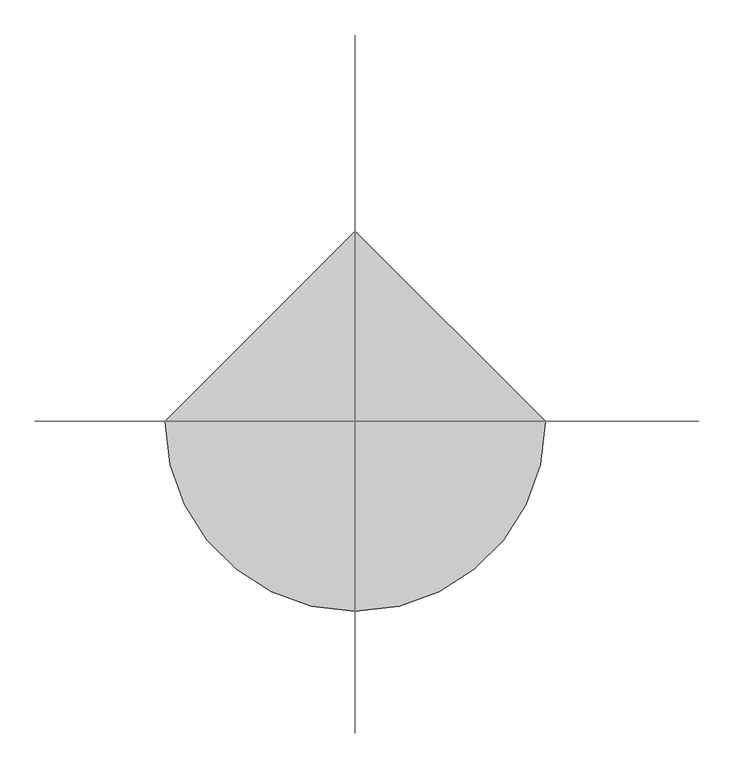
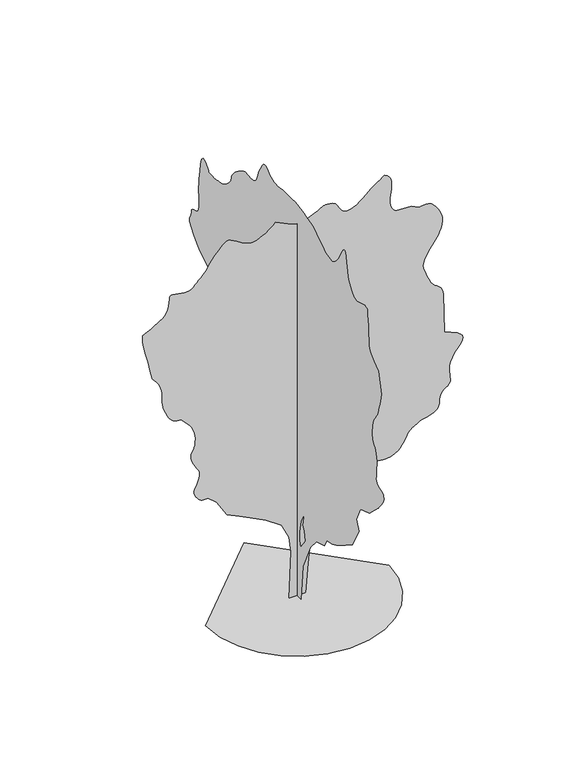
"""IFC4 building model written with IfcOpenShell, lengths in millimetres: geographic element geometry, RPC 木 - 落葉樹 : アメリカサイカチ - 7.6 メートル."""

from ifc_helpers import new_model, si_unit, origin, place, context, project, spatial, triangles, source, transform, mapped, element, save


def geographic_element_4d039a6d(model_context):
    return source(origin(), model_context, "Body", "Tessellation", [
        triangles([(0.0017518, 137.8833715, 0.0), (0.0017518, -126.6771787, 0.0), (0.0017518, -184.1906286, 667.1526644), (0.0017518, -425.7465056, 1173.2690826), (0.0017518, -609.7879246, 1391.8195507), (0.0017518, -862.844862, 1472.3389091), (0.0017518, -931.8629602, 1610.3700188), (0.0017518, -1115.9043428, 1656.3802917), (0.0017518, -1165.0661676, 1674.6229282), (0.0017518, -1231.7358627, 1707.9563587), (0.0017518, -1312.9923855, 1753.8679459), (0.0017518, -1405.9175274, 1809.8393841), (0.0017518, -1507.5978035, 1873.3551292), (0.0017518, -1615.1123165, 1941.9019627), (0.0017518, -1725.5454014, 2012.9618694), (0.0017518, -1932.5919205, 2392.5485836), (0.0017518, -1852.072562, 2576.5999947), (0.0017518, -1978.6023388, 2841.1559395), (0.0017518, -2266.1682163, 2944.6676445), (0.0017518, -2530.7289574, 3197.7222565), (0.0017518, -2537.2320488, 3205.5755562), (0.0017518, -2554.6106392, 3226.7033363), (0.0017518, -2579.6146362, 3257.4834343), (0.0017518, -2609.0773727, 3294.3181046), (0.0017518, -2639.7307343, 3333.559314), (0.0017518, -2668.3574753, 3371.5846092), (0.0017518, -2691.7653488, 3404.7712463), (0.0017518, -2707.3199226, 3435.5004753), (0.0017518, -2714.843882, 3467.42062), (0.0017518, -2714.6918564, 3498.9605553), (0.0017518, -2707.3199226, 3528.4485809), (0.0017518, -2693.1079994, 3554.3391518), (0.0017518, -2672.4612946, 3575.0111458), (0.0017518, -2645.7600174, 3588.8178612), (0.0017518, -2614.4732643, 3598.8750961), (0.0017518, -2581.3627853, 3610.1482452), (0.0017518, -2548.8601181, 3623.8285149), (0.0017518, -2519.3950562, 3641.1309471), (0.0017518, -2495.3485588, 3663.2723282), (0.0017518, -2479.1504196, 3691.4429924), (0.0017518, -2473.2147354, 3726.8588539), (0.0017518, -2475.0617157, 3770.3056206), (0.0017518, -2479.5204552, 3821.0228737), (0.0017518, -2484.9872726, 3877.7694099), (0.0017518, -2489.8486038, 3939.3293152), (0.0017518, -2492.4984421, 4004.5372536), (0.0017518, -2491.3255486, 4072.1267326), (0.0017518, -2484.7186844, 4140.9571243), (0.0017518, -2471.0692268, 4202.6943443), (0.0017518, -2451.5852417, 4251.7396065), (0.0017518, -2428.8815403, 4290.9558174), (0.0017518, -2405.5749687, 4323.1035645), (0.0017518, -2384.2797569, 4351.0463356), (0.0017518, -2367.6128963, 4377.570298), (0.0017518, -2358.1889076, 4405.5130692), (0.0017518, -2353.3934155, 4438.4462334), (0.0017518, -2349.4033974, 4477.4089714), (0.0017518, -2347.022002, 4521.4126808), (0.0017518, -2347.0549942, 4569.4446327), (0.0017518, -2350.307848, 4620.465937), (0.0017518, -2357.5860374, 4673.5138618), (0.0017518, -2369.6928566, 4727.5753876), (0.0017518, -2385.7895485, 4775.3791557), (0.0017518, -2404.1004948, 4812.695192), (0.0017518, -2424.0200638, 4843.1712387), (0.0017518, -2444.9455307, 4870.4550385), (0.0017518, -2466.2735893, 4898.1190475), (0.0017518, -2487.4013695, 4929.8112991), (0.0017518, -2507.7239662, 4969.1280853), (0.0017518, -2527.4434021, 5018.1989273), (0.0017518, -2547.162838, 5075.7053009), (0.0017518, -2566.8721001, 5140.2804291), (0.0017518, -2586.6066513, 5210.4534714), (0.0017518, -2606.3162041, 5284.8826492), (0.0017518, -2626.0254662, 5362.0988663), (0.0017518, -2645.7600174, 5440.7585999), (0.0017518, -2542.2227325, 5820.3272919), (0.0017518, -2404.1993259, 5923.8645767), (0.0017518, -2369.9284527, 5951.1995361), (0.0017518, -2337.0635983, 5979.8262772), (0.0017518, -2307.015723, 6011.0871597), (0.0017518, -2281.193462, 6046.2751282), (0.0017518, -2261.0053047, 6086.6819641), (0.0017518, -2247.8574154, 6133.6244476), (0.0017518, -2243.1630798, 6188.4205215), (0.0017518, -2241.8229, 6252.9444901), (0.0017518, -2238.0660072, 6327.120195), (0.0017518, -2232.2976093, 6409.3523849), (0.0017518, -2224.9205887, 6498.0190659), (0.0017518, -2216.3350662, 6591.5238235), (0.0017518, -2206.9440697, 6688.2214096), (0.0017518, -2197.1528069, 6786.5654068), (0.0017518, -2179.7816288, 6796.2427231), (0.0017518, -2161.706424, 6804.9317276), (0.0017518, -2142.2225842, 6811.6196915), (0.0017518, -2120.6259373, 6815.2677246), (0.0017518, -2096.2121658, 6814.8880966), (0.0017518, -2068.2770977, 6809.4919144), (0.0017518, -2036.1165607, 6798.066449), (0.0017518, -2001.6074753, 6783.4743164), (0.0017518, -1967.1010059, 6770.0983887), (0.0017518, -1932.5919205, 6759.1292908), (0.0017518, -1898.082835, 6751.7826462), (0.0017518, -1863.5763657, 6749.2746597), (0.0017518, -1829.0674255, 6752.7959564), (0.0017518, -1794.5608109, 6763.5627411), (0.0017518, -1761.0576233, 6783.7027908), (0.0017518, -1729.3681332, 6813.5195755), (0.0017518, -1699.1859638, 6851.3934265), (0.0017518, -1670.2098255, 6895.6756073), (0.0017518, -1642.1404633, 6944.8226074), (0.0017518, -1614.6765873, 6997.1612732), (0.0017518, -1587.5116756, 7051.1207703), (0.0017518, -1518.4962662, 7465.2193314), (0.0017518, -1506.0550198, 7474.5925964), (0.0017518, -1492.9096012, 7481.1794037), (0.0017518, -1478.3555477, 7482.1165558), (0.0017518, -1461.6888325, 7474.5925964), (0.0017518, -1442.2049927, 7455.8204865), (0.0017518, -1419.1997108, 7422.9631897), (0.0017518, -1391.9689602, 7373.1830887), (0.0017518, -1362.8939907, 7316.7406036), (0.0017518, -1334.019009, 7265.3396713), (0.0017518, -1304.1384201, 7218.371608), (0.0017518, -1272.0461929, 7175.2033127), (0.0017518, -1236.5315002, 7135.2528442), (0.0017518, -1196.3882383, 7097.9370987), (0.0017518, -1150.4133556, 7062.6223938), (0.0017518, -1098.0975809, 7039.1889404), (0.0017518, -1040.3503063, 7035.6676437), (0.0017518, -978.073439, 7048.7395203), (0.0017518, -912.1764439, 7075.0861679), (0.0017518, -843.5636988, 7111.414183), (0.0017518, -773.1396544, 7154.3795837), (0.0017518, -701.8086159, 7200.6633865), (0.0017518, -657.5437305, 7232.507373), (0.0017518, -613.8792446, 7263.2618912), (0.0017518, -571.4231515, 7291.8124741), (0.0017518, -530.778394, 7317.019075), (0.0017518, -492.5479151, 7337.8178055), (0.0017518, -457.3371283, 7353.0686188), (0.0017518, -425.7465056, 7361.6820465), (0.0017518, -378.7962828, 7372.2459366), (0.0017518, -303.6779573, 7391.2715195), (0.0017518, -210.2471958, 7414.5020782), (0.0017518, -108.3667684, 7437.7576355), (0.0017518, -7.8945933, 7456.7576385), (0.0017518, 81.3095355, 7467.32211), (0.0017518, 149.3864666, 7465.2193314), (0.0017518, 203.5460423, 7458.5057877), (0.0017518, 257.3028083, 7456.6314835), (0.0017518, 310.2544999, 7457.365741), (0.0017518, 362.0002876, 7458.5057877), (0.0017518, 412.1349092, 7457.8471069), (0.0017518, 460.2580619, 7453.1351852), (0.0017518, 505.9669724, 7442.2166656), (0.0017518, 554.0242498, 7432.1085617), (0.0017518, 607.3128576, 7430.4621506), (0.0017518, 662.6104271, 7435.8833313), (0.0017518, 716.7045816, 7446.9030075), (0.0017518, 766.3705908, 7462.1538208), (0.0017518, 808.3909184, 7480.2416702), (0.0017518, 839.5433046, 7499.7230392), (0.0017518, 867.4124611, 7523.4099655), (0.0017518, 900.5129843, 7551.0989731), (0.0017518, 937.0309587, 7576.9898346), (0.0017518, 975.1626429, 7595.2300003), (0.0017518, 1013.0891069, 7599.9925003), (0.0017518, 1049.006682, 7585.4259476), (0.0017518, 1081.0989092, 7545.7283707), (0.0017518, 1108.6666306, 7497.2656311), (0.0017518, 1132.6091372, 7458.075), (0.0017518, 1153.5370022, 7424.7113388), (0.0017518, 1172.0480089, 7393.7539261), (0.0017518, 1188.7477163, 7361.7832031), (0.0017518, 1204.2416107, 7325.4046097), (0.0017518, 1219.1324896, 7281.1730072), (0.0017518, 1233.4508743, 7235.9275131), (0.0017518, 1247.7718025, 7198.1304016), (0.0017518, 1263.4987495, 7166.7927795), (0.0017518, 1282.0426758, 7140.8513397), (0.0017518, 1304.8148323, 7119.3689301), (0.0017518, 1333.2184765, 7101.2810806), (0.0017518, 1368.6648594, 7085.6250595), (0.0017518, 1409.9809422, 7076.5302658), (0.0017518, 1454.1141495, 7076.3023727), (0.0017518, 1499.6558464, 7081.0904526), (0.0017518, 1545.1949272, 7087.0941559), (0.0017518, 1589.3281345, 7090.4887161), (0.0017518, 1630.6442173, 7087.4487854), (0.0017518, 1667.7346859, 7074.123436), (0.0017518, 1709.8209251, 7049.7528305), (0.0017518, 1763.5782543, 7017.1234268), (0.0017518, 1823.7753067, 6977.8316391), (0.0017518, 1885.1780994, 6933.548877), (0.0017518, 1942.5580273, 6885.8209763), (0.0017518, 1990.6812527, 6836.2943481), (0.0017518, 2024.3162636, 6786.5654068), (0.0017518, 2042.2243275, 6744.8162109), (0.0017518, 2050.6755558, 6714.5174789), (0.0017518, 2055.7041733, 6690.2730286), (0.0017518, 2063.3523983, 6666.637262), (0.0017518, 2079.6492233, 6638.1628372), (0.0017518, 2110.6370121, 6599.4279922), (0.0017518, 2162.3473732, 6545.0121277), (0.0017518, 2224.3226601, 6490.849736), (0.0017518, 2282.0700073, 6453.9897766), (0.0017518, 2335.5915951, 6430.6069016), (0.0017518, 2384.887714, 6416.9013428), (0.0017518, 2429.9608349, 6409.0227539), (0.0017518, 2470.8055801, 6403.145787), (0.0017518, 2507.4274727, 6395.4695114), (0.0017518, 2546.8082085, 6388.2240234), (0.0017518, 2592.8135399, 6385.4125671), (0.0017518, 2640.819912, 6385.817775), (0.0017518, 2686.2427208, 6388.2240234), (0.0017518, 2724.3947525, 6391.4418503), (0.0017518, 2750.6905312, 6394.2538879), (0.0017518, 2760.4945839, 6395.4695114), (0.0017518, 2772.097364, 6413.5829407), (0.0017518, 2802.5984093, 6455.8390823), (0.0017518, 2845.5890991, 6504.1239258), (0.0017518, 2894.6343613, 6540.3507843), (0.0017518, 2943.2491264, 6546.3800674), (0.0017518, 2985.0489006, 6504.1239258), (0.0017518, 3013.5489052, 6395.4695114), (0.0017518, 3031.2062576, 6264.7751633), (0.0017518, 3045.0635513, 6164.0749146), (0.0017518, 3055.5009956, 6086.7069626), (0.0017518, 3062.8982185, 6026.0339218), (0.0017518, 3067.7115875, 5975.4434052), (0.0017518, 3070.2957321, 5928.2474487), (0.0017518, 3071.0555695, 5877.8592453), (0.0017518, 3069.8396553, 5823.6206955), (0.0017518, 3067.0276176, 5769.4077255), (0.0017518, 3063.8103722, 5715.1691757), (0.0017518, 3061.4035423, 5660.9306259), (0.0017518, 3060.9983345, 5606.7170746), (0.0017518, 3063.8103722, 5552.4785248), (0.0017518, 3071.0555695, 5498.2649734), (0.0017518, 3091.0435936, 5455.4263092), (0.0017518, 3126.7382172, 5430.3214462), (0.0017518, 3171.2488724, 5415.2735275), (0.0017518, 3217.8114372, 5402.6318573), (0.0017518, 3259.5353439, 5384.7469025), (0.0017518, 3289.580603, 5353.991803), (0.0017518, 3301.107225, 5302.7176071), (0.0017518, 3309.9741257, 5250.3027832), (0.0017518, 3329.6833878, 5214.3799759), (0.0017518, 3350.0007523, 5184.7149261), (0.0017518, 3360.6660896, 5150.9960541), (0.0017518, 3351.4192703, 5103.0146805), (0.0017518, 3311.975457, 5030.4853867), (0.0017518, 3232.0995186, 4923.1233353), (0.0017518, 3129.6769913, 4811.4284088), (0.0017518, 3031.0795212, 4728.0820427), (0.0017518, 2938.7145195, 4666.2939537), (0.0017518, 2855.0132332, 4619.1741554), (0.0017518, 2782.3824921, 4579.9073662), (0.0017518, 2723.2294167, 4541.6288887), (0.0017518, 2679.9599648, 4497.5234413), (0.0017518, 2651.1814888, 4453.0636551), (0.0017518, 2631.471936, 4415.0383598), (0.0017518, 2617.1841454, 4378.6088974), (0.0017518, 2604.7200806, 4338.9877693), (0.0017518, 2590.4319992, 4291.2851578), (0.0017518, 2570.697448, 4230.7129829), (0.0017518, 2541.9442612, 4152.4584572), (0.0017518, 2511.1159103, 4067.4145203), (0.0017518, 2486.9380257, 3989.0079689), (0.0017518, 2468.290036, 3916.1240456), (0.0017518, 2454.0728806, 3847.6735725), (0.0017518, 2443.1747086, 3782.5667908), (0.0017518, 2434.4878841, 3719.6389458), (0.0017518, 2426.9081142, 3657.8511475), (0.0017518, 2448.9074982, 3633.0497543), (0.0017518, 2469.7998276, 3607.462944), (0.0017518, 2488.4780479, 3580.2803009), (0.0017518, 2503.8378662, 3550.6658295), (0.0017518, 2514.7715012, 3517.8338219), (0.0017518, 2520.1700089, 3480.9738625), (0.0017518, 2518.9314217, 3439.3005341), (0.0017518, 2519.7342796, 3398.0327042), (0.0017518, 2526.7771637, 3361.425927), (0.0017518, 2532.2085182, 3327.0233757), (0.0017518, 2528.185508, 3292.3926407), (0.0017518, 2506.8574493, 3255.1780518), (0.0017518, 2460.3759842, 3212.9222008), (0.0017518, 2380.8976959, 3163.2182579), (0.0017518, 2293.371207, 3122.7861328), (0.0017518, 2224.3556522, 3103.0515816), (0.0017518, 2168.4172062, 3093.8047623), (0.0017518, 2120.1268398, 3084.7608376), (0.0017518, 2074.0481117, 3065.6343887), (0.0017518, 2024.7519928, 3026.1902847), (0.0017518, 1966.8020416, 2956.1689774), (0.0017518, 1913.8857948, 2878.471685), (0.0017518, 1880.0810268, 2819.0904259), (0.0017518, 1860.5617241, 2772.3758354), (0.0017518, 1850.501873, 2732.7038383), (0.0017518, 1845.0703732, 2694.4253609), (0.0017518, 1839.4362694, 2651.9413261), (0.0017518, 1828.770932, 2599.6026604), (0.0017518, 1818.5767868, 2549.4935097), (0.0017518, 1813.4114044, 2514.2825775), (0.0017518, 1807.039991, 2489.1317871), (0.0017518, 1793.2232471, 2469.2120728), (0.0017518, 1765.7239082, 2449.6929153), (0.0017518, 1718.3051456, 2425.7503361), (0.0017518, 1644.7295494, 2392.5485836), (0.0017518, 1563.1714462, 2360.7247993), (0.0017518, 1493.6873154, 2340.7697674), (0.0017518, 1432.8519299, 2327.6598118), (0.0017518, 1377.2503819, 2316.3561413), (0.0017518, 1323.4602058, 2301.8375507), (0.0017518, 1268.058791, 2279.0653942), (0.0017518, 1207.628686, 2243.0161411), (0.0017518, 1141.8659122, 2196.3015507), (0.0017518, 1073.0860262, 2145.3587299), (0.0017518, 1001.7879072, 2090.8998447), (0.0017518, 928.4809719, 2033.6212189), (0.0017518, 853.6640997, 1974.2297859), (0.0017518, 777.8389315, 1913.4298634), (0.0017518, 701.5122677, 1851.9256233), (0.0017518, 275.9151897, 1529.8506603), (0.0017518, 149.3864666, 1311.3001923), (0.0017518, 114.8781896, 1138.7626133), (0.0017518, 103.3756032, 874.2017996), (0.0020698, -103.6720059, 977.7238237), (0.0020698, -80.666824, 1104.2535278), (0.0020698, -80.666824, 1265.2897739), (0.0020698, -126.6771787, 1495.3440456), (0.0020698, -230.2009742, 1702.3907101), (0.0020698, -184.1906286, 1449.3337727), (0.0020698, -230.2009742, 1368.8144142), (0.0020698, -264.7077343, 1196.2742918), (154.3819466, 0.0004423, 0.01624), (-144.686372, 0.0004423, 0.01624), (-110.1786128, 0.0003915, 874.2169876), (-144.686372, 0.000377, 1161.7829378), (-282.7171909, 0.0003625, 1437.8450844), (-558.7818446, 0.000348, 1633.390416), (-961.3737316, 0.0003335, 1840.4395512), (-1260.4435581, 0.0003262, 1978.4705154), (-1455.9887444, 0.0003118, 2289.0416748), (-1605.5211868, 0.0002973, 2415.5714516), (-1632.5847965, 0.0003045, 2413.2888874), (-1659.3468258, 0.0003045, 2412.1159939), (-1685.5035141, 0.0003045, 2413.1545933), (-1710.7557518, 0.0002973, 2417.5145016), (-1734.799633, 0.0002973, 2426.3026279), (-1757.3360481, 0.0002973, 2440.6210854), (-1778.0612366, 0.0002973, 2461.5817245), (-1798.1835548, 0.0002973, 2486.9327934), (-1817.9005199, 0.0002973, 2513.6948227), (-1835.4057014, 0.00029, 2541.868103), (-1848.8881634, 0.00029, 2571.4319962), (-1856.5337723, 0.00029, 2602.4399872), (-1856.5337723, 0.00029, 2634.815918), (-1847.0767914, 0.0002828, 2668.6359467), (-1828.7658451, 0.0002828, 2707.0667404), (-1806.2319008, 0.0002828, 2752.1346291), (-1783.6954857, 0.0002755, 2802.0411758), (-1765.3845394, 0.0002755, 2854.9623642), (-1755.5248215, 0.0002683, 2909.0744682), (-1758.3418007, 0.0002683, 2962.603759), (-1778.0612366, 0.0002683, 3013.7009308), (-1808.0432728, 0.000261, 3061.7075935), (-1837.6199558, 0.000261, 3107.4850319), (-1864.9850006, 0.0002538, 3151.6407669), (-1888.3270351, 0.0002538, 3194.8087715), (-1905.832362, 0.0002538, 3237.5459885), (-1915.6896091, 0.0002465, 3280.5113892), (-1916.0923462, 0.0002465, 3324.2872055), (-1908.6140236, 0.0002465, 3361.8058456), (-1897.1126907, 0.0002393, 3389.2672508), (-1883.1944996, 0.0002393, 3412.1178909), (-1868.4733051, 0.0002393, 3435.7539482), (-1854.5552593, 0.0002393, 3465.6218925), (-1843.0513103, 0.0002393, 3507.1684845), (-1835.5754585, 0.000232, 3565.8404846), (-1834.3341099, 0.0002248, 3630.8202393), (-1839.7327629, 0.0002248, 3688.5803764), (-1850.6640724, 0.0002248, 3740.2856506), (-1866.0236, 0.0002175, 3787.1775558), (-1884.7044365, 0.0002175, 3830.4214279), (-1905.5967659, 0.0002175, 3871.28405), (-1927.5961498, 0.0002103, 3910.9054688), (-2088.6323959, 0.000203, 4083.4504601), (-2125.5887157, 0.000203, 4083.931826), (-2162.4435883, 0.000203, 4087.1999405), (-2199.0983276, 0.000203, 4096.1171288), (-2235.4516319, 0.000203, 4113.4960098), (-2271.3995831, 0.0001958, 4142.1477493), (-2306.8484367, 0.0001958, 4184.8596771), (-2341.6919495, 0.0001885, 4244.4944092), (-2372.7454319, 0.0001885, 4310.259581), (-2397.1592033, 0.0001813, 4370.5782829), (-2415.3333847, 0.0001813, 4427.0969261), (-2427.6756546, 0.0001813, 4481.3860542), (-2434.5840992, 0.000174, 4535.0673706), (-2436.4613102, 0.000174, 4589.7619972), (-2433.7126408, 0.0001668, 4647.0913467), (-2433.5100368, 0.0001668, 4705.4340065), (-2441.9611198, 0.0001595, 4761.7753349), (-2457.8552078, 0.0001595, 4815.5072296), (-2479.9916473, 0.0001523, 4865.9965897), (-2507.1539429, 0.0001523, 4912.6856003), (-2538.1442024, 0.0001523, 4954.9417419), (-2571.7360474, 0.000145, 4992.1563309), (-2599.27332, 0.000145, 5022.9870071), (-2615.9426514, 0.000145, 5051.3858551), (-2626.3800957, 0.000145, 5084.8256744), (-2635.1961273, 0.0001378, 5130.7292679), (-2647.0268005, 0.0001378, 5196.5705978), (-2666.5078789, 0.0001305, 5289.7468872), (-2698.2759979, 0.0001233, 5417.7559341), (-2732.3492088, 0.000116, 5550.2240112), (-2756.7706833, 0.0001088, 5654.9263412), (-2773.1359634, 0.0001015, 5736.4742706), (-2783.0411728, 0.0001015, 5799.5291428), (-2788.158593, 9.43e-05, 5848.70056), (-2790.0331879, 9.43e-05, 5888.6010315), (-2790.2866608, 9.43e-05, 5923.8645767), (-2772.7557541, 9.43e-05, 5931.4646942), (-2753.5025688, 9.43e-05, 5940.1287003), (-2730.8292435, 8.7e-05, 5951.0472198), (-2703.0384979, 8.7e-05, 5965.2591431), (-2668.3827644, 8.7e-05, 5983.9045166), (-2625.1894707, 8.7e-05, 6008.0728088), (-2571.7360474, 8.7e-05, 6038.9034851), (-2516.0737473, 7.98e-05, 6070.5189972), (-2467.2462044, 7.98e-05, 6098.9178452), (-2425.0588085, 7.98e-05, 6127.949794), (-2389.3109905, 7.98e-05, 6161.3646149), (-2359.8001465, 7.25e-05, 6203.0632324), (-2336.3262886, 7.25e-05, 6256.8204163), (-2318.686813, 6.53e-05, 6326.4615143), (-2308.0543224, 6.53e-05, 6395.8241409), (-2302.6558147, 5.8e-05, 6447.4535477), (-2297.8601772, 5.8e-05, 6483.4013535), (-2289.039204, 5.8e-05, 6505.6697617), (-2271.5693401, 5.8e-05, 6516.28423), (-2240.8172928, 5.8e-05, 6517.2213821), (-2192.1570362, 5.8e-05, 6510.5084198), (-2134.475528, 5.8e-05, 6500.3241577), (-2080.0140266, 5.8e-05, 6490.9253128), (-2029.175124, 5.8e-05, 6484.5414001), (-1982.3592316, 5.8e-05, 6483.4013535), (-1939.9715572, 5.8e-05, 6489.7096893), (-1902.4123672, 5.8e-05, 6505.6697617), (-1870.0819279, 5.8e-05, 6533.5110855), (-1839.6997707, 5.08e-05, 6565.8108582), (-1807.3034924, 5.08e-05, 6596.0840103), (-1772.2928387, 5.08e-05, 6627.9785751), (-1734.0624687, 5.08e-05, 6665.1175873), (-1692.0090763, 4.35e-05, 6711.0973389), (-1645.5300819, 4.35e-05, 6769.5414459), (-1594.019854, 3.63e-05, 6844.0973602), (-1542.1397358, 2.9e-05, 6920.5025803), (-1494.4853771, 2.9e-05, 6983.658609), (-1450.3546406, 2.9e-05, 7035.7438019), (-1409.0385578, 2.18e-05, 7078.9620941), (-1369.8352821, 2.18e-05, 7115.5435822), (-1332.0404961, 2.18e-05, 7147.7166183), (-1294.9500275, 1.45e-05, 7177.6607208), (-1284.6900433, 1.45e-05, 7189.5925507), (-1272.0132008, 1.45e-05, 7199.2192886), (-1254.5078739, 1.45e-05, 7204.2352615), (-1229.7573498, 1.45e-05, 7202.2847992), (-1195.3496389, 1.45e-05, 7191.0872269), (-1148.8705719, 1.45e-05, 7168.3130356), (-1087.9034357, 2.18e-05, 7131.6553894), (-1024.0508652, 2.18e-05, 7090.8945053), (-968.6519938, 2.18e-05, 7057.8087341), (-918.8846827, 2.9e-05, 7032.9567627), (-871.9344961, 2.9e-05, 7016.9716919), (-824.9867804, 2.9e-05, 7010.4104645), (-775.2194693, 2.9e-05, 7013.9317612), (-719.8180544, 2.9e-05, 7028.1181046), (-663.0106934, 2.18e-05, 7050.1836182), (-610.4263304, 2.18e-05, 7076.4796875), (-561.3633004, 2.18e-05, 7106.2970535), (-515.1173587, 2.18e-05, 7138.9264572), (-470.9867311, 1.45e-05, 7173.683638), (-428.2621224, 1.45e-05, 7209.8343384), (-386.2417585, 1.45e-05, 7246.668718), (-167.6915448, 2.18e-05, 7143.1570129), (-133.0495187, 2.18e-05, 7126.1074722), (-97.6028996, 2.18e-05, 7110.4008728), (-60.5463543, 2.18e-05, 7097.278418), (-21.0752102, 2.18e-05, 7088.0824677), (21.6153412, 2.18e-05, 7084.1303833), (68.3302632, 2.18e-05, 7086.7145279), (119.8741692, 2.18e-05, 7097.1516815), (179.4667345, 2.18e-05, 7116.9371017), (245.9002885, 2.18e-05, 7144.1703232), (313.3401037, 1.45e-05, 7175.0259979), (375.9513619, 1.45e-05, 7205.654361), (427.8973191, 1.45e-05, 7232.27948), (463.3436657, 1.45e-05, 7251.0765884), (476.4562011, 1.45e-05, 7258.1703415), (486.2475002, 1.45e-05, 7260.3486969), (512.5409534, 1.45e-05, 7264.3513596), (550.7030499, 1.45e-05, 7266.3274017), (596.1104527, 1.45e-05, 7262.476474), (644.1322672, 1.45e-05, 7248.9488113), (690.1426128, 1.45e-05, 7221.9690628), (729.5131021, 1.45e-05, 7177.6607208), (759.026417, 2.18e-05, 7129.5020325), (781.0917852, 2.18e-05, 7092.41418), (799.536953, 2.18e-05, 7064.7757507), (818.1822538, 2.18e-05, 7044.9903305), (840.8530357, 2.9e-05, 7031.437088), (871.3695597, 2.9e-05, 7022.5196091), (913.5571009, 2.9e-05, 7016.6170624), (965.3687639, 2.9e-05, 7020.9237762), (1021.0032314, 2.18e-05, 7041.1144043), (1078.6517475, 2.18e-05, 7073.3635986), (1136.5003241, 2.18e-05, 7113.8715912), (1192.7377344, 1.45e-05, 7158.8130341), (1245.5576935, 1.45e-05, 7204.361998), (1293.1437424, 1.45e-05, 7246.668718), (1336.8412205, 7.3e-06, 7284.1112), (1379.3301968, 7.3e-06, 7317.9062302), (1420.8135658, 7.3e-06, 7348.6857468), (1461.4911701, 7.3e-06, 7377.0590149), (1501.5659042, 0.0, 7403.634137), (1541.2379013, 0.0, 7428.9674744), (1580.7097652, 0.0, 7453.7177078), (1607.6390808, 0.0, 7440.9754623), (1633.4613419, 0.0, 7425.724649), (1657.0693485, 0.0, 7405.4328644), (1677.3588078, 7.3e-06, 7377.5915405), (1693.2200489, 7.3e-06, 7339.7182709), (1703.550959, 7.3e-06, 7289.2289108), (1707.239542, 1.45e-05, 7223.6660522), (1704.1538292, 2.18e-05, 7154.3795837), (1696.6425144, 2.18e-05, 7093.3513321), (1687.319973, 2.18e-05, 7038.9610474), (1678.8002895, 2.9e-05, 6989.5861542), (1673.7032169, 2.9e-05, 6943.6569809), (1674.6431305, 3.63e-05, 6899.526535), (1684.2342602, 3.63e-05, 6855.5984024), (1699.0239098, 3.63e-05, 6815.9264053), (1713.8109432, 4.35e-05, 6784.6905212), (1728.6005928, 4.35e-05, 6760.5228104), (1743.390097, 4.35e-05, 6741.9785934), (1758.1797466, 4.35e-05, 6727.6399338), (1772.9667801, 4.35e-05, 6716.1388916), (1787.7562843, 4.35e-05, 6706.0557861), (2063.8209743, 4.35e-05, 6694.554744), (2201.852084, 5.08e-05, 6625.5467468), (2211.6788097, 5.08e-05, 6628.4093628), (2238.2053883, 5.08e-05, 6634.5148041), (2277.0033108, 5.08e-05, 6640.0121429), (2323.6520622, 5.08e-05, 6641.1016113), (2373.7208084, 5.08e-05, 6633.9322815), (2422.783802, 5.08e-05, 6614.6788055), (2466.412825, 5.08e-05, 6579.5158356), (2506.0848221, 5.8e-05, 6531.8135147), (2544.3508003, 5.8e-05, 6478.0563309), (2578.3987221, 6.53e-05, 6419.2575943), (2605.3787613, 6.53e-05, 6356.4561951), (2622.5294586, 7.25e-05, 6290.6148651), (2626.9879074, 7.25e-05, 6222.7724945), (2615.9426514, 7.98e-05, 6153.9162323), (2595.220079, 7.98e-05, 6089.5951584), (2572.6987793, 8.7e-05, 6033.7351959), (2548.632225, 8.7e-05, 5984.9178268), (2523.3898705, 8.7e-05, 5941.7245331), (2497.2307114, 9.43e-05, 5902.7367966), (2470.4712982, 9.43e-05, 5866.5860962), (2443.4078339, 9.43e-05, 5831.8539139), (2401.8914726, 0.0001015, 5770.3448776), (2362.6881969, 0.0001015, 5709.5451004), (2328.1132725, 0.0001088, 5650.1638412), (2300.4796394, 0.0001088, 5592.8853607), (2282.1028542, 0.000116, 5538.4183365), (2275.2958569, 0.000116, 5487.4731903), (2282.3714424, 0.0001233, 5440.7585999), (2297.226931, 0.0001233, 5397.6158844), (2312.4851566, 0.0001233, 5356.0440033), (2328.5490017, 0.0001305, 5314.9029099), (2345.8187325, 0.0001305, 5272.9508194), (2364.6997021, 0.0001305, 5228.9976883), (2385.5920315, 0.0001378, 5181.8017319), (2408.8986031, 0.0001378, 5130.1973236), (2439.1490822, 0.000145, 5084.0402573), (2477.6481857, 0.000145, 5049.7644424), (2519.9674049, 0.000145, 5020.9348068), (2561.6788124, 0.000145, 4991.0924423), (2598.3867462, 0.0001523, 4953.8016953), (2625.5946785, 0.0001523, 4902.628656), (2638.9453171, 0.0001595, 4831.1123817), (2661.9479828, 0.000203, 4094.9517929), (2891.9996384, 0.0002103, 3991.4400879), (2928.251786, 0.0002103, 3968.8679192), (2960.1969292, 0.0002103, 3943.9906586), (2983.4530678, 0.0002103, 3914.4773438), (2993.7637756, 0.0002103, 3878.0228828), (2986.7464714, 0.0002175, 3832.2960228), (2958.1197304, 0.0002175, 3775.0175423), (2903.5009712, 0.0002248, 3703.8561882), (2843.3092964, 0.000232, 3627.7044411), (2799.4317421, 0.000232, 3556.5683762), (2769.8172707, 0.0002393, 3489.8657616), (2752.4639694, 0.0002393, 3426.9884949), (2745.3957962, 0.0002465, 3367.3287643), (2746.561132, 0.0002465, 3310.303466), (2753.9839348, 0.0002538, 3255.2542099), (2762.2171532, 0.0002538, 3205.702002), (2766.4479996, 0.0002538, 3164.3835938), (2765.4599785, 0.000261, 3129.7022804), (2758.0118866, 0.000261, 3100.0622292), (2742.9133896, 0.000261, 3073.842318), (2718.9732811, 0.000261, 3049.4208435), (2684.9506485, 0.000261, 3025.2022636), (2649.6106544, 0.0002683, 2999.8183479), (2621.9213562, 0.0002683, 2972.8383087), (2601.0467583, 0.0002683, 2944.0089638), (2586.2267326, 0.0002683, 2913.2038673), (2576.6508636, 0.0002755, 2880.1692558), (2571.4828651, 0.0002755, 2844.7278145), (2569.9373199, 0.0002755, 2806.6519409), (2567.7333847, 0.0002828, 2769.2600372), (2560.6907913, 0.0002828, 2735.6931908), (2548.2014374, 0.0002828, 2705.5464844), (2529.6929741, 0.0002828, 2678.4147102), (2504.541893, 0.00029, 2653.9173683), (2472.1482307, 0.00029, 2631.5986725), (2431.9038849, 0.00029, 2611.1039932), (2390.0860886, 0.00029, 2595.1442116), (2352.2914478, 0.00029, 2584.8335037), (2316.9109039, 0.00029, 2577.3095444), (2282.3359795, 0.00029, 2569.8108742), (2246.9580517, 0.00029, 2559.4748772), (2209.1632656, 0.00029, 2543.5148048), (2167.3429985, 0.0002973, 2519.0936211), (2128.7782013, 0.0002973, 2495.0825867), (2099.6702396, 0.0002973, 2479.1201889), (2076.7992519, 0.0002973, 2466.5776405), (2056.9455219, 0.0002973, 2452.8290611), (2036.8916588, 0.0002973, 2433.2439194), (2013.4178009, 0.0003045, 2403.1961895), (1983.3016159, 0.0003045, 2358.0572296), (1952.2479881, 0.0003045, 2304.6697906), (1925.0172375, 0.0003118, 2253.4939899), (1896.9808674, 0.0003118, 2205.3379177), (1863.5129974, 0.000319, 2161.0021065), (1819.9854218, 0.000319, 2121.2972626), (1761.7668823, 0.000319, 2087.0237732), (1684.2342602, 0.000319, 2058.9874031), (1607.0690575, 0.0003262, 2044.3346638), (1548.6175381, 0.0003262, 2044.5676437), (1502.2372295, 0.000319, 2052.0461117), (1461.291037, 0.000319, 2059.1216972), (1419.136488, 0.000319, 2058.1514076), (1369.1360516, 0.0003262, 2041.4820763), (1304.6450752, 0.0003262, 2001.4757973), (1232.8480042, 0.0003262, 1952.4456505), (1165.4740643, 0.0003335, 1912.0694813), (1102.7284756, 0.0003335, 1877.7301529), (1044.8139874, 0.0003335, 1846.8108192), (991.9281893, 0.0003335, 1816.6946342), (944.2762287, 0.0003408, 1784.769548), (902.0532246, 0.0003408, 1748.4162437), (861.274173, 0.0003408, 1708.6429447), (818.0808792, 0.000348, 1668.2667755), (772.876153, 0.000348, 1627.3888927), (726.0601879, 0.000348, 1586.1058022), (678.0358664, 0.0003553, 1544.5211311), (629.2084688, 0.0003553, 1502.736327), (579.9807687, 0.0003553, 1460.8502209), (338.4251278, 0.000377, 1173.2842707), (234.9010689, 0.0003915, 897.2221968), (200.3922923, 0.0004133, 540.6406554), (-1654.2371086, 0.0, 0.0171681), (-1610.5043129, -379.0420163, 0.0171681), (-1485.9555199, -727.1317795, 0.0171681), (-1290.5597431, -1034.2956614, 0.0171681), (-1034.2956614, -1290.5597431, 0.0171681), (-727.1317795, -1485.9555199, 0.0171681), (-379.0420163, -1610.5043129, 0.0171681), (7.23e-05, -1654.2371086, 0.0171681), (379.0420163, -1610.5043129, 0.0171681), (727.1317795, -1485.9555199, 0.0171681), (1034.2956614, -1290.5597431, 0.0171681), (1290.5597431, -1034.2956614, 0.0171681), (1485.9555199, -727.1317795, 0.0171681), (1610.5043129, -379.0420163, 0.0171681), (1654.2371086, 0.000145, 0.0171681), (-0.0002169, 1654.2371086, 0.0171681)], [[328, 1, 329], [327, 328, 329], [327, 329, 330], [329, 1, 2], [329, 2, 3], [329, 3, 4], [336, 329, 4], [327, 330, 331], [326, 327, 331], [326, 331, 332], [325, 326, 332], [335, 336, 4], [335, 4, 5], [325, 332, 333], [334, 335, 5], [333, 334, 5], [333, 5, 6], [333, 6, 7], [324, 325, 333], [91, 92, 93], [223, 224, 225], [222, 223, 225], [222, 225, 226], [221, 222, 226], [220, 221, 226], [220, 226, 227], [219, 220, 227], [219, 227, 228], [15, 16, 17], [91, 93, 94], [91, 94, 95], [91, 95, 96], [91, 96, 97], [91, 97, 98], [91, 98, 99], [91, 99, 100], [90, 91, 100], [90, 100, 101], [90, 101, 102], [89, 90, 102], [89, 102, 103], [88, 89, 103], [88, 103, 104], [218, 219, 228], [14, 15, 17], [218, 228, 229], [217, 218, 229], [216, 217, 229], [216, 229, 230], [215, 216, 230], [215, 230, 231], [214, 215, 231], [214, 231, 232], [214, 232, 233], [214, 233, 234], [213, 214, 234], [213, 234, 235], [113, 114, 115], [113, 115, 116], [113, 116, 117], [113, 117, 118], [113, 118, 119], [113, 119, 120], [113, 120, 121], [113, 121, 122], [113, 122, 123], [113, 123, 124], [113, 124, 125], [113, 125, 126], [113, 126, 127], [112, 113, 127], [112, 127, 128], [111, 112, 128], [110, 111, 128], [213, 235, 236], [87, 88, 104], [87, 104, 105], [212, 213, 236], [110, 128, 129], [109, 110, 129], [212, 236, 237], [211, 212, 237], [210, 211, 237], [86, 87, 105], [210, 237, 238], [209, 210, 238], [85, 86, 105], [76, 77, 78], [75, 76, 78], [13, 14, 17], [209, 238, 239], [85, 105, 106], [208, 209, 239], [74, 75, 78], [108, 109, 129], [74, 78, 79], [73, 74, 79], [84, 85, 106], [73, 79, 80], [72, 73, 80], [71, 72, 80], [208, 239, 240], [70, 71, 80], [69, 70, 80], [68, 69, 80], [67, 68, 80], [66, 67, 80], [65, 66, 80], [65, 80, 81], [64, 65, 81], [12, 13, 17], [245, 246, 247], [244, 245, 247], [243, 244, 247], [243, 247, 248], [64, 81, 82], [63, 64, 82], [242, 243, 248], [323, 324, 333], [167, 168, 169], [167, 169, 170], [166, 167, 170], [166, 170, 171], [165, 166, 171], [164, 165, 171], [164, 171, 172], [163, 164, 172], [163, 172, 173], [163, 173, 174], [162, 163, 174], [162, 174, 175], [162, 175, 176], [162, 176, 177], [161, 162, 177], [161, 177, 178], [161, 178, 179], [160, 161, 179], [160, 179, 180], [159, 160, 180], [159, 180, 181], [158, 159, 181], [11, 12, 17], [250, 251, 252], [249, 250, 252], [249, 252, 253], [248, 249, 253], [242, 248, 253], [242, 253, 254], [242, 254, 255], [241, 242, 255], [241, 255, 256], [241, 256, 257], [241, 257, 258], [241, 258, 259], [240, 241, 259], [208, 240, 259], [208, 259, 260], [208, 260, 261], [207, 208, 261], [206, 207, 261], [206, 261, 262], [206, 262, 263], [205, 206, 263], [205, 263, 264], [204, 205, 264], [204, 264, 265], [204, 265, 266], [204, 266, 267], [204, 267, 268], [204, 268, 269], [203, 204, 269], [10, 11, 17], [9, 10, 17], [8, 9, 17], [7, 8, 17], [333, 7, 17], [323, 333, 17], [322, 323, 17], [322, 17, 18], [321, 322, 18], [320, 321, 18], [319, 320, 18], [318, 319, 18], [317, 318, 18], [316, 317, 18], [315, 316, 18], [203, 269, 270], [314, 315, 18], [18, 19, 20], [314, 18, 20], [314, 20, 21], [314, 21, 22], [314, 22, 23], [314, 23, 24], [314, 24, 25], [314, 25, 26], [314, 26, 27], [314, 27, 28], [314, 28, 29], [314, 29, 30], [314, 30, 31], [314, 31, 32], [314, 32, 33], [314, 33, 34], [314, 34, 35], [314, 35, 36], [314, 36, 37], [314, 37, 38], [314, 38, 39], [314, 39, 40], [314, 40, 41], [314, 41, 42], [314, 42, 43], [314, 43, 44], [314, 44, 45], [314, 45, 46], [314, 46, 47], [314, 47, 48], [314, 48, 49], [314, 49, 50], [314, 50, 51], [314, 51, 52], [314, 52, 53], [314, 53, 54], [314, 54, 55], [314, 55, 56], [314, 56, 57], [314, 57, 58], [314, 58, 59], [314, 59, 60], [314, 60, 61], [314, 61, 62], [313, 314, 62], [312, 313, 62], [311, 312, 62], [310, 311, 62], [309, 310, 62], [308, 309, 62], [307, 308, 62], [306, 307, 62], [305, 306, 62], [304, 305, 62], [303, 304, 62], [302, 303, 62], [301, 302, 62], [300, 301, 62], [299, 300, 62], [298, 299, 62], [297, 298, 62], [296, 297, 62], [295, 296, 62], [294, 295, 62], [294, 62, 63], [294, 63, 82], [294, 82, 83], [294, 83, 84], [294, 84, 106], [294, 106, 107], [294, 107, 108], [294, 108, 129], [294, 129, 130], [294, 130, 131], [294, 131, 132], [294, 132, 133], [294, 133, 134], [294, 134, 135], [294, 135, 136], [294, 136, 137], [294, 137, 138], [294, 138, 139], [294, 139, 140], [294, 140, 141], [294, 141, 142], [294, 142, 143], [294, 143, 144], [294, 144, 145], [294, 145, 146], [294, 146, 147], [294, 147, 148], [294, 148, 149], [294, 149, 150], [294, 150, 151], [294, 151, 152], [294, 152, 153], [294, 153, 154], [294, 154, 155], [294, 155, 156], [294, 156, 157], [294, 157, 158], [294, 158, 181], [294, 181, 182], [294, 182, 183], [294, 183, 184], [294, 184, 185], [293, 294, 185], [293, 185, 186], [293, 186, 187], [292, 293, 187], [292, 187, 188], [292, 188, 189], [292, 189, 190], [292, 190, 191], [292, 191, 192], [292, 192, 193], [292, 193, 194], [292, 194, 195], [292, 195, 196], [292, 196, 197], [292, 197, 198], [292, 198, 199], [292, 199, 200], [292, 200, 201], [292, 201, 202], [292, 202, 203], [292, 203, 270], [292, 270, 271], [292, 271, 272], [292, 272, 273], [292, 273, 274], [292, 274, 275], [291, 292, 275], [290, 291, 275], [289, 290, 275], [289, 275, 276], [289, 276, 277], [289, 277, 278], [289, 278, 279], [289, 279, 280], [289, 280, 281], [289, 281, 282], [289, 282, 283], [288, 289, 283], [288, 283, 284], [287, 288, 284], [286, 287, 284], [285, 286, 284], [337, 338, 339], [677, 337, 339], [676, 677, 339], [676, 339, 340], [675, 676, 340], [423, 424, 425], [486, 487, 488], [675, 340, 341], [674, 675, 341], [529, 530, 531], [485, 486, 488], [484, 485, 488], [423, 425, 426], [529, 531, 532], [673, 674, 341], [673, 341, 342], [672, 673, 342], [671, 672, 342], [670, 671, 342], [669, 670, 342], [668, 669, 342], [667, 668, 342], [529, 532, 533], [528, 529, 533], [528, 533, 534], [528, 534, 535], [528, 535, 536], [527, 528, 536], [527, 536, 537], [526, 527, 537], [526, 537, 538], [525, 526, 538], [525, 538, 539], [524, 525, 539], [524, 539, 540], [523, 524, 540], [523, 540, 541], [522, 523, 541], [522, 541, 542], [521, 522, 542], [521, 542, 543], [520, 521, 543], [519, 520, 543], [519, 543, 544], [519, 544, 545], [518, 519, 545], [518, 545, 546], [517, 518, 546], [517, 546, 547], [422, 423, 426], [422, 426, 427], [441, 442, 443], [441, 443, 444], [440, 441, 444], [440, 444, 445], [439, 440, 445], [439, 445, 446], [438, 439, 446], [438, 446, 447], [438, 447, 448], [437, 438, 448], [437, 448, 449], [666, 667, 342], [421, 422, 427], [421, 427, 428], [421, 428, 429], [420, 421, 429], [420, 429, 430], [419, 420, 430], [419, 430, 431], [418, 419, 431], [418, 431, 432], [418, 432, 433], [417, 418, 433], [417, 433, 434], [416, 417, 434], [483, 484, 488], [436, 437, 449], [343, 344, 345], [666, 342, 343], [666, 343, 345], [665, 666, 345], [664, 665, 345], [663, 664, 345], [662, 663, 345], [661, 662, 345], [660, 661, 345], [659, 660, 345], [659, 345, 346], [517, 547, 548], [483, 488, 489], [416, 434, 435], [415, 416, 435], [482, 483, 489], [482, 489, 490], [436, 449, 450], [658, 659, 346], [414, 415, 435], [600, 601, 602], [599, 600, 602], [599, 602, 603], [598, 599, 603], [597, 598, 603], [597, 603, 604], [596, 597, 604], [596, 604, 605], [596, 605, 606], [596, 606, 607], [596, 607, 608], [516, 517, 548], [516, 548, 549], [413, 414, 435], [412, 413, 435], [411, 412, 435], [410, 411, 435], [409, 410, 435], [408, 409, 435], [407, 408, 435], [407, 435, 436], [407, 436, 450], [407, 450, 451], [406, 407, 451], [405, 406, 451], [405, 451, 452], [404, 405, 452], [404, 452, 453], [404, 453, 454], [404, 454, 455], [404, 455, 456], [551, 552, 553], [482, 490, 491], [481, 482, 491], [404, 456, 457], [467, 468, 469], [467, 469, 470], [466, 467, 470], [466, 470, 471], [466, 471, 472], [465, 466, 472], [465, 472, 473], [464, 465, 473], [463, 464, 473], [463, 473, 474], [462, 463, 474], [461, 462, 474], [461, 474, 475], [460, 461, 475], [459, 460, 475], [459, 475, 476], [458, 459, 476], [458, 476, 477], [457, 458, 477], [404, 457, 477], [404, 477, 478], [404, 478, 479], [404, 479, 480], [403, 404, 480], [403, 480, 481], [403, 481, 491], [403, 491, 492], [403, 492, 493], [402, 403, 493], [401, 402, 493], [400, 401, 493], [399, 400, 493], [398, 399, 493], [397, 398, 493], [396, 397, 493], [395, 396, 493], [394, 395, 493], [393, 394, 493], [392, 393, 493], [391, 392, 493], [390, 391, 493], [389, 390, 493], [388, 389, 493], [387, 388, 493], [386, 387, 493], [386, 493, 494], [385, 386, 494], [384, 385, 494], [384, 494, 495], [383, 384, 495], [383, 495, 496], [383, 496, 497], [382, 383, 497], [382, 497, 498], [382, 498, 499], [382, 499, 500], [381, 382, 500], [381, 500, 501], [381, 501, 502], [381, 502, 503], [381, 503, 504], [381, 504, 505], [381, 505, 506], [381, 506, 507], [381, 507, 508], [381, 508, 509], [381, 509, 510], [381, 510, 511], [381, 511, 512], [381, 512, 513], [381, 513, 514], [381, 514, 515], [381, 515, 516], [381, 516, 549], [381, 549, 550], [381, 550, 551], [381, 551, 553], [380, 381, 553], [379, 380, 553], [378, 379, 553], [378, 553, 554], [378, 554, 555], [378, 555, 556], [378, 556, 557], [378, 557, 558], [378, 558, 559], [378, 559, 560], [378, 560, 561], [378, 561, 562], [378, 562, 563], [378, 563, 564], [378, 564, 565], [378, 565, 566], [378, 566, 567], [378, 567, 568], [378, 568, 569], [378, 569, 570], [378, 570, 571], [378, 571, 572], [378, 572, 573], [378, 573, 574], [378, 574, 575], [378, 575, 576], [378, 576, 577], [378, 577, 578], [378, 578, 579], [378, 579, 580], [378, 580, 581], [378, 581, 582], [378, 582, 583], [378, 583, 584], [378, 584, 585], [378, 585, 586], [378, 586, 587], [378, 587, 588], [378, 588, 589], [378, 589, 590], [378, 590, 591], [378, 591, 592], [378, 592, 593], [378, 593, 594], [378, 594, 595], [378, 595, 596], [378, 596, 608], [378, 608, 609], [378, 609, 610], [378, 610, 611], [378, 611, 612], [378, 612, 613], [378, 613, 614], [378, 614, 615], [378, 615, 616], [378, 616, 617], [378, 617, 618], [378, 618, 619], [378, 619, 620], [378, 620, 621], [378, 621, 622], [378, 622, 623], [378, 623, 624], [378, 624, 625], [378, 625, 626], [378, 626, 627], [378, 627, 628], [378, 628, 629], [378, 629, 630], [378, 630, 631], [378, 631, 632], [378, 632, 633], [378, 633, 634], [378, 634, 635], [378, 635, 636], [378, 636, 637], [378, 637, 638], [378, 638, 639], [378, 639, 640], [378, 640, 641], [378, 641, 642], [378, 642, 643], [378, 643, 644], [378, 644, 645], [378, 645, 646], [378, 646, 647], [378, 647, 648], [378, 648, 649], [378, 649, 650], [378, 650, 651], [378, 651, 652], [378, 652, 653], [378, 653, 654], [378, 654, 655], [378, 655, 656], [378, 656, 657], [378, 657, 658], [378, 658, 346], [377, 378, 346], [358, 359, 360], [357, 358, 360], [356, 357, 360], [356, 360, 361], [355, 356, 361], [354, 355, 361], [354, 361, 362], [353, 354, 362], [352, 353, 362], [351, 352, 362], [350, 351, 362], [349, 350, 362], [348, 349, 362], [347, 348, 362], [346, 347, 362], [346, 362, 363], [346, 363, 364], [346, 364, 365], [346, 365, 366], [377, 346, 366], [377, 366, 367], [377, 367, 368], [377, 368, 369], [377, 369, 370], [377, 370, 371], [377, 371, 372], [377, 372, 373], [377, 373, 374], [377, 374, 375], [377, 375, 376], [692, 693, 678], [691, 692, 678], [691, 678, 679], [690, 691, 679], [690, 679, 680], [690, 680, 681], [689, 690, 681], [688, 689, 681], [688, 681, 682], [688, 682, 683], [688, 683, 684], [688, 684, 685], [688, 685, 686], [688, 686, 687]], closed=False),
    ])


if __name__ == "__main__":
    model = new_model("IFC4")
    model_context = context("Model", 3, world=origin())
    ifc_project = project(units=[si_unit("LENGTHUNIT", "METRE", prefix="MILLI")], contexts=[model_context])
    site = spatial("IfcSite", under=ifc_project)
    building = spatial("IfcBuilding", under=site)
    placement = place(None, origin())
    geographic_element_shape = geographic_element_4d039a6d(model_context)
    element("IfcGeographicElement", 1, ObjectType="RPC 木 - 落葉樹 : アメリカサイカチ - 7.6 メートル", at=placement, inside=building, context=model_context, shape_type="MappedRepresentation", body=[
        mapped(geographic_element_shape, transform((0.0, 0.0, 0.0), x_axis=(1.0, 0.0, 0.0), y_axis=(0.0, 1.0, 0.0), z_axis=(0.0, 0.0, 1.0))),
    ])
    save(model, "model.ifc")

# Revit data of these elements
# Type "RPC 木 - 落葉樹 : アメリカサイカチ - 7.6 メートル"
#   built-in parameter 1005198 = "{2, 15},{39, RPC-16-G2VH-N100-5X50-0000-ST1L-LVER-AU},{1, 0},{1, 0},{2, 35},{1, 8},{5, Color},{1, 0},{1, 0},{3, 0.8},{3, 0.8},{3, 0.8},{1, 8},{7, BBoxMin},{1, 0},{1, 0},{1, 0},{1, 0},{1, 0},{1, 8},{7, BBoxMax},{1, 0},{1, 0},{1, 0},{1, 0},{1, 0},{2, 11},{9, RPCTypeId},{1, 0},{1, 0},{39, RPC-16-G2VH-N100-5X50-0000-ST1L-LVER-AU},{1, 6},{14, RPCPlantHeight},{1, 0},{1, 0},{7, 24.9344},{2, 11},{7, keyword},{1, 0},{1, 0},{224, :Geometry:RPC:Honey-Locust:Gleditsia triacanthos L.  Rare in Canada; occurs in southwestern Ontario; commonly planted beyond its range because of its tolerance to droughty and alkaline soils; frequently becoming naturalized.},{2, 11},{8, category},{1, 0},{1, 0},{16, :Trees [General]},{2, 11},{12, LocalizedUID},{1, 0},{1, 0},{12, Honey-Locust},{2, 14},{6, Height},{1, 0},{1, 0},{7, 24.9344},{1, 2},{16, Cast Reflections},{1, 0},{1, 0},{1, 0},{1, 2},{12, Cast Shadows},{1, 0},{1, 0},{1, 1},{1, 2},{9, Lock View},{1, 0},{1, 0},{1, 0},{1, 4},{5, ViewC},{1, 0},{1, 0},{1, 0},{2, 11},{20, AdvancedUIDefinition},{1, 0},{1, 0},{0, },{2, 11},{10, AssetLibID},{1, 0},{1, 0},{36, 4D3F6E72-3F99-4203-98E9-AF80B3C7A7A4},{2, 11},{10, BaseSchema},{1, 0},{1, 0},{9, RPCSchema},{2, 11},{12, ExchangeGUID},{1, 0},{1, 0},{0, },{1, 2},{6, Hidden},{1, 0},{1, 0},{1, 0},{1, 4},{11, RPCCategory},{1, 0},{1, 0},{1, 0},{2, 11},{8, RPCImage},{1, 0},{1, 0},{0, },{1, 4},{13, SchemaVersion},{1, 0},{1, 0},{1, 4},{2, 11},{12, UIDefinition},{1, 0},{1, 0},{0, },{2, 11},{6, UIName},{1, 0},{1, 0},{39, RPC-16-G2VH-N100-5X50-0000-ST1L-LVER-AU},{2, 11},{11, VersionGUID},{1, 0},{1, 0},{9, RPCSchema},{2, 11},{9, assettype},{1, 0},{1, 0},{11, RPCGeometry},{2, 11},{11, description},{1, 0},{1, 0},{0, },{2, 11},{9, localname},{1, 0},{1, 0},{3, RPC},{2, 11},{9, localtype},{1, 0},{1, 0},{3, RPC},{1, 4},{8, revision},{1, 0},{1, 0},{1, 1},{2, 11},{9, thumbnail},{1, 0},{1, 0},{0, },{1, 4},{7, version},{1, 0},{1, 0},{1, 1},{1, 2},{20, RPC_Cast Reflections},{1, 0},{1, 0},{1, 1},{1, 2},{16, RPC_Cast Shadows},{1, 0},{1, 0},{1, 1},{1, 2},{13, RPC_Lock View},{1, 0},{1, 0},{1, 0},{1, 4},{9, RPC_ViewC},{1, 0},{1, 0},{1, 0},{21, assetlibrary_base.fbx},{1, 5},"
#   built-in parameter 1005195 = "RPC-16-G2VH-N100-5X50-0000-ST1L-LVER-AU"
#   Type Comments = "アメリカサイカチ"
#   Height = 7600 mm
#   Default Elevation = 0
